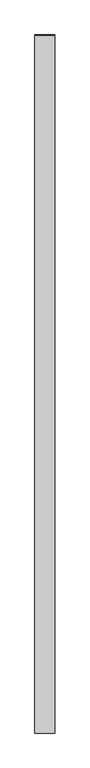
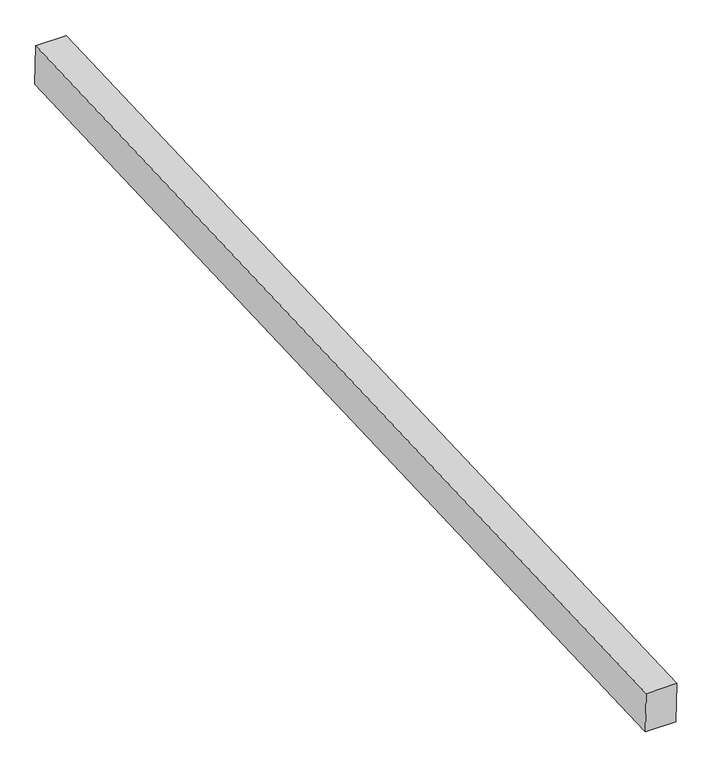
"""IFC4 building model written with IfcOpenShell, lengths in millimetres: proxy geometry, Generic Models 7:Generic Models 1:8:Generic Models 1:8 : Generic Models 7:Generic Models 1:337419:50 : Generic Models 7:Generic Models 1:8:Generic Models 1:8 : Generic Models 7:Generic Models 1:337419:315935."""

from ifc_helpers import new_model, si_unit, frame, origin, place, context, project, spatial, polyline, outline, extrude, source, transform, mapped, element, save


def generic_models_d38a3f58(model_context):
    return source(origin(), model_context, "Body", "SweptSolid", [
        extrude(outline(polyline([(-581229.2495411, 3818.908703), (-576356.3266468, 4021.9471569), (-576348.7597251, 3831.5971524), (-581221.3189223, 3628.5738526), (-581229.2495411, 3818.908703)])), frame((615724.961724, 0.0, 0.0), z_axis=(1.0, 0.0, 0.0), x_axis=(0.0, 1.0, 0.0)), (0.0, 0.0, 1.0), 139.7),
    ])


if __name__ == "__main__":
    model = new_model("IFC4")
    model_context = context("Model", 3, world=origin())
    ifc_project = project(units=[si_unit("LENGTHUNIT", "METRE", prefix="MILLI")], contexts=[model_context])
    site = spatial("IfcSite", under=ifc_project)
    building = spatial("IfcBuilding", under=site)
    placement = place(None, origin())
    generic_models_shape = generic_models_d38a3f58(model_context)
    element("IfcBuildingElementProxy", 1, Name="Generic Models 7:Generic Models 1:8:Generic Models 1:8 : Generic Models 7:Generic Models 1:337419:50 : Generic Models 7:Generic Models 1:8:Generic Models 1:8 : Generic Models 7:Generic Models 1:337419:315935", ObjectType="Generic Models 7:Generic Models 1:8:Generic Models 1:8 : Generic Models 7:Generic Models 1:337419:50 : Generic Models 7:Generic Models 1:8:Generic Models 1:8 : Generic Models 7:Generic Models 1:337419:315935", at=placement, inside=building, context=model_context, shape_type="MappedRepresentation", body=[
        mapped(generic_models_shape, transform((0.0, 0.0, 0.0), x_axis=(1.0, 0.0, 0.0), y_axis=(0.0, 1.0, 0.0), z_axis=(0.0, 0.0, 1.0))),
    ])
    save(model, "model.ifc")

# Revit data of these elements
# Type "Generic Models 7:Generic Models 1:8:Generic Models 1:8 : Generic Models 7:Generic Models 1:337419:50 : Generic Models 7:Generic Models 1:8:Generic Models 1:8 : Generic Models 7:Generic Models 1:337419:315935"
#   NameOverride = "Generic Models 7:Generic Models 1:8:Generic Models 1:8 : Generic Models 7:Generic Models 1:337419:315935"
#   ObjectTypeOverride = "Generic Models 1:8 : Generic Models 7:Generic Models 1:337419"
#   Reference = "Generic Models 1"
#   Tag = "315935"
# Element 1 (IfcBuildingElementProxy, "Generic Models 7:Generic Models 1:8:Generic Models 1:8 : Generic Models 7:Generic Models 1:337419:50 : Generic Models 7:Generic Models 1:8:Generic Models 1:8 : Generic Models 7:Generic Models 1:337419:315935")
#   Materials on its faces: "5 1/2\" X 7 1/2\" EXTERIOR GRADE GLULAM BEAMS"
# Materials
#   "5 1/2\" X 7 1/2\" EXTERIOR GRADE GLULAM BEAMS": class "Wood", colour RGB 183 134 68, transparency 0, Keynote = "M06181300.01", Description = "Pinus Echinata", Cost = 0
